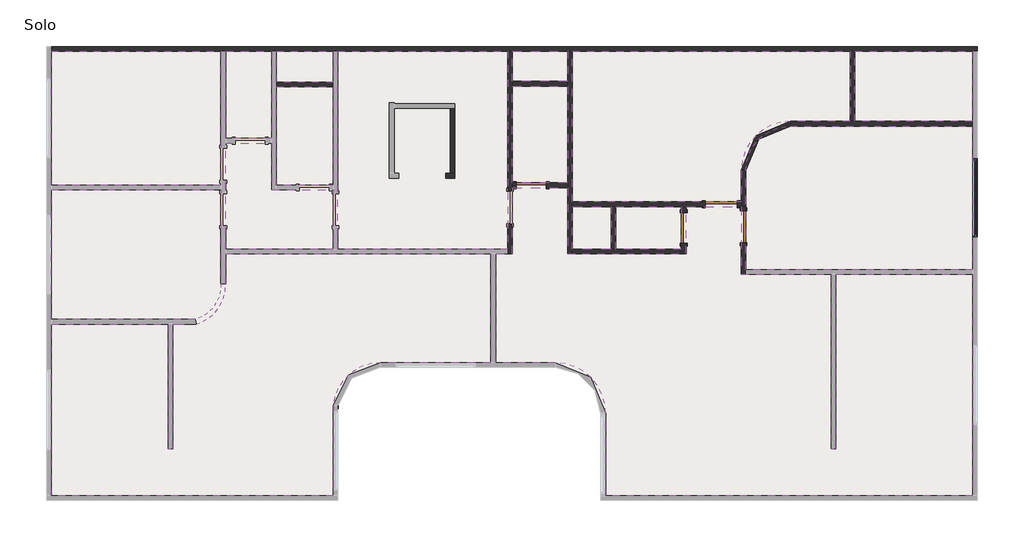
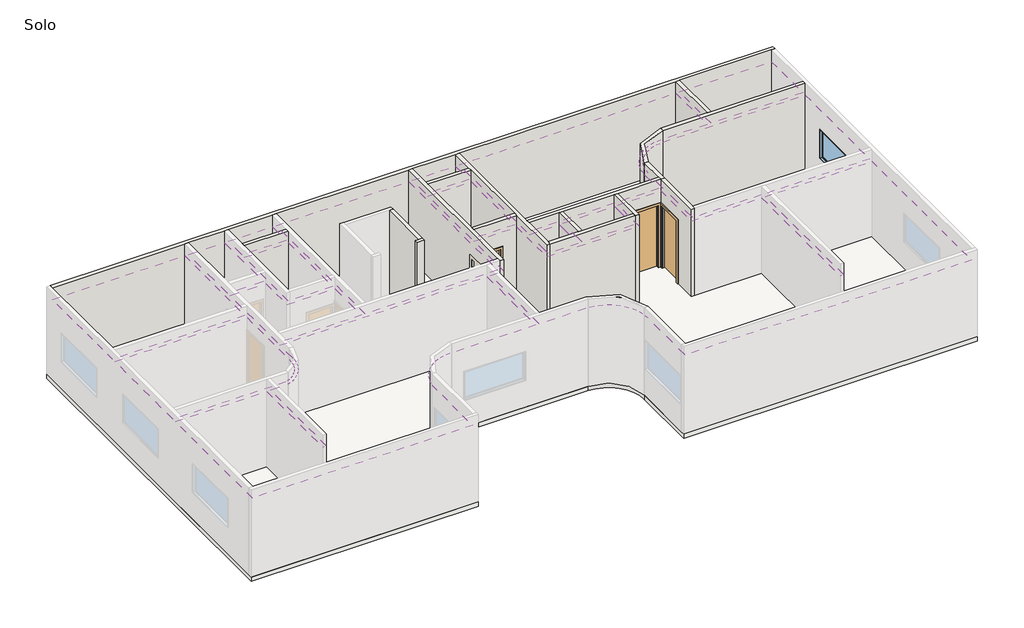
# One storey, part 2 of 2: 17 walls, 16 coverings, 4 doors, 1 slab, 1 window.
"""IFC4 building model written with IfcOpenShell, lengths in millimetres."""

import ifcopenshell
import ifcopenshell.guid

model = None  # the IFC model being written
_history = None  # IfcOwnerHistory: only IFC2X3 demands one
_inside = {}  # id of a spatial element -> (the spatial element, [elements in it])
_under = {}  # id of a project, library or spatial element -> (it, [spatial elements below it])
_declared = {}  # id of a project -> (the project, [libraries it declares])
_typed = {}  # id of a type object -> (the type object, [elements of that type])
_made_of = {}  # id of a material, layer set ... -> (it, [elements and type objects made of it])


def new_model(schema):
    """Start an empty IFC model of exactly this schema.

    Asked for "IFC4X3", IfcOpenShell would pick the latest addendum, in which some entities
    have other attributes; the version numbers below select the first issue.
    IFC2X3 requires an IfcOwnerHistory on every rooted entity: one is made here for all.
    """
    global model, _history
    if schema == "IFC4X3":
        model = ifcopenshell.file(schema_version=(4, 3, 0, 0))
    else:
        model = ifcopenshell.file(schema=schema)
    _inside.clear()
    _under.clear()
    _declared.clear()
    _typed.clear()
    _made_of.clear()
    _history = None
    if model.schema == "IFC2X3":
        org = make("IfcOrganization", Name="unknown")
        user = make(
            "IfcPersonAndOrganization",
            ThePerson=make("IfcPerson", FamilyName="unknown"),
            TheOrganization=org,
        )
        app = make(
            "IfcApplication",
            ApplicationDeveloper=org,
            Version="unknown",
            ApplicationFullName="unknown",
            ApplicationIdentifier="unknown",
        )
        _history = make(
            "IfcOwnerHistory",
            OwningUser=user,
            OwningApplication=app,
            ChangeAction="ADDED",
            CreationDate=0,
        )
    return model


def make(cls, **values):
    """One entity of the class cls with the attributes given. An attribute that is None is left unset."""
    return model.create_entity(
        cls, **{name: value for name, value in values.items() if value is not None}
    )


def rooted(cls, **values):
    """An entity with a GlobalId (a new one), such as an element, a storey or a relation."""
    return make(cls, GlobalId=ifcopenshell.guid.new(), OwnerHistory=_history, **values)


def si_unit(unit_type, name, prefix=None):
    """IfcSIUnit, for example si_unit("LENGTHUNIT", "METRE", prefix="MILLI")."""
    return make("IfcSIUnit", UnitType=unit_type, Prefix=prefix, Name=name)


def assignment(units):
    """IfcUnitAssignment: the units of a project."""
    return None if units is None else make("IfcUnitAssignment", Units=units)


def point(xyz):
    """IfcCartesianPoint."""
    return None if xyz is None else make("IfcCartesianPoint", Coordinates=xyz)


def direction(xyz):
    """IfcDirection."""
    return None if xyz is None else make("IfcDirection", DirectionRatios=xyz)


def frame(location, z_axis=None, x_axis=None):
    """IfcAxis2Placement3D, a coordinate frame: its origin and axes. An axis left out is left unset."""
    return make(
        "IfcAxis2Placement3D",
        Location=point(location),
        Axis=direction(z_axis),
        RefDirection=direction(x_axis),
    )


def frame_2d(location, x_axis=None):
    """IfcAxis2Placement2D, a coordinate frame in the plane: its origin and x axis."""
    return make(
        "IfcAxis2Placement2D", Location=point(location), RefDirection=direction(x_axis)
    )


def origin():
    """The frame at (0, 0, 0) with its axes left unset."""
    return frame((0.0, 0.0, 0.0))


def origin_with_axes():
    """The frame at (0, 0, 0) with the z axis (0, 0, 1) and the x axis (1, 0, 0) written out."""
    return frame((0.0, 0.0, 0.0), z_axis=(0.0, 0.0, 1.0), x_axis=(1.0, 0.0, 0.0))


def place(relative_to, where):
    """IfcLocalPlacement: puts the frame where relative to a parent placement (None: the world)."""
    return make(
        "IfcLocalPlacement", PlacementRelTo=relative_to, RelativePlacement=where
    )


def context(
    kind, dimensions, precision=None, world=None, true_north=None, identifier=None
):
    """IfcGeometricRepresentationContext, for example the 3D "Model" context."""
    return make(
        "IfcGeometricRepresentationContext",
        ContextIdentifier=identifier,
        ContextType=kind,
        CoordinateSpaceDimension=dimensions,
        Precision=precision,
        WorldCoordinateSystem=world,
        TrueNorth=true_north,
    )


def project(units=None, contexts=None):
    """IfcProject with its units and contexts."""
    return rooted(
        "IfcProject",
        Name="project",
        RepresentationContexts=contexts,
        UnitsInContext=assignment(units),
    )


def spatial(cls, under=None, at=None, **own):
    """A site, building, storey or space (cls), placed at a placement, below another one or the project."""
    s = rooted(cls, ObjectPlacement=at, **own)
    if under is not None:
        _under.setdefault(under.id(), (under, []))[1].append(s)
    return s


def polyline(points):
    """IfcPolyline through the points."""
    return make("IfcPolyline", Points=[point(p) for p in points])


def circle_curve(where, radius):
    """IfcCircle in the frame where."""
    return make("IfcCircle", Position=where, Radius=radius)


def trimmed(basis, trim1, trim2, sense, master):
    """IfcTrimmedCurve: the piece of a basis curve between two trims."""
    return make(
        "IfcTrimmedCurve",
        BasisCurve=basis,
        Trim1=trim1,
        Trim2=trim2,
        SenseAgreement=sense,
        MasterRepresentation=master,
    )


def segment(curve, same_sense, transition):
    """IfcCompositeCurveSegment."""
    return make(
        "IfcCompositeCurveSegment",
        Transition=transition,
        SameSense=same_sense,
        ParentCurve=curve,
    )


def composite_curve(segments, self_intersect=None):
    """IfcCompositeCurve: segments joined end to end."""
    return make("IfcCompositeCurve", Segments=segments, SelfIntersect=self_intersect)


def outline(outer, holes=None, kind="AREA"):
    """IfcArbitraryClosedProfileDef: a profile drawn as a closed curve; with holes, ...WithVoids."""
    if holes is None:
        return make("IfcArbitraryClosedProfileDef", ProfileType=kind, OuterCurve=outer)
    return make(
        "IfcArbitraryProfileDefWithVoids",
        ProfileType=kind,
        OuterCurve=outer,
        InnerCurves=holes,
    )


def extrude(swept, where, along, depth):
    """IfcExtrudedAreaSolid: the profile swept, set in the frame where, extruded along a direction by depth."""
    return make(
        "IfcExtrudedAreaSolid",
        SweptArea=swept,
        Position=where,
        ExtrudedDirection=direction(along),
        Depth=depth,
    )


def faces_of(points, faces, orient=None, outer=None):
    """IfcFace entities. A face is a list of loops; a loop is a list of indices into points, from 0.

    orient and outer hold one flag for each loop. By default every Orientation is true, the
    first loop of a face is its IfcFaceOuterBound and the others are IfcFaceBound.
    """
    made = []
    for i, loops in enumerate(faces):
        bounds = []
        for j, loop in enumerate(loops):
            is_outer = j == 0 if outer is None else outer[i][j]
            bounds.append(
                make(
                    "IfcFaceOuterBound" if is_outer else "IfcFaceBound",
                    Bound=make("IfcPolyLoop", Polygon=[points[k] for k in loop]),
                    Orientation=True if orient is None else orient[i][j],
                )
            )
        made.append(make("IfcFace", Bounds=bounds))
    return made


def faceted_brep(points, faces, orient=None, outer=None, voids=None):
    """IfcFacetedBrep: a solid bounded by flat faces; with voids (closed shells), ...WithVoids."""
    shared = [point(p) for p in points]
    hull = make("IfcClosedShell", CfsFaces=faces_of(shared, faces, orient, outer))
    if voids is None:
        return make("IfcFacetedBrep", Outer=hull)
    return make(
        "IfcFacetedBrepWithVoids",
        Outer=hull,
        Voids=[
            make(cls, CfsFaces=faces_of(shared, fs, o, b)) for cls, fs, o, b in voids
        ],
    )


def shape(context_of_items, identifier, shape_type, items):
    """IfcShapeRepresentation: the items that make up one representation, for example the "Body"."""
    return make(
        "IfcShapeRepresentation",
        ContextOfItems=context_of_items,
        RepresentationIdentifier=identifier,
        RepresentationType=shape_type,
        Items=items,
    )


def source(mapping_origin, context_of_items, identifier, shape_type, items):
    """IfcRepresentationMap: a shape defined once, which mapped items show again and again."""
    return make(
        "IfcRepresentationMap",
        MappingOrigin=mapping_origin,
        MappedRepresentation=shape(context_of_items, identifier, shape_type, items),
    )


def transform(
    local_origin,
    x_axis=None,
    y_axis=None,
    z_axis=None,
    scale=None,
    scale2=None,
    scale3=None,
    uniform=True,
):
    """IfcCartesianTransformationOperator3D, or its non-uniform kind. x_axis, y_axis, z_axis: its Axis1, 2, 3."""
    if uniform:
        return make(
            "IfcCartesianTransformationOperator3D",
            Axis1=direction(x_axis),
            Axis2=direction(y_axis),
            LocalOrigin=point(local_origin),
            Scale=scale,
            Axis3=direction(z_axis),
        )
    return make(
        "IfcCartesianTransformationOperator3DnonUniform",
        Axis1=direction(x_axis),
        Axis2=direction(y_axis),
        LocalOrigin=point(local_origin),
        Scale=scale,
        Axis3=direction(z_axis),
        Scale2=scale2,
        Scale3=scale3,
    )


def mapped(mapping_source, mapping_target):
    """IfcMappedItem: shows the shape of a source again, moved by a transform."""
    return make(
        "IfcMappedItem", MappingSource=mapping_source, MappingTarget=mapping_target
    )


def made_of(thing, what):
    """Note that an element or type object is made of a material, layer set ...; save() writes the relation."""
    if what is not None:
        _made_of.setdefault(what.id(), (what, []))[1].append(thing)
    return thing


def element(
    cls,
    number,
    at=None,
    inside=None,
    cuts=None,
    type_object=None,
    material=None,
    context=None,
    identifier="Body",
    shape_type=None,
    held_by="IfcProductDefinitionShape",
    body=None,
    shapes=None,
    **own,
):
    """One element of the class cls, such as IfcWall. Its Tag is "e" and its number.

    at: its placement. inside: the storey or other place that contains it. cuts: it is an
    opening in that element (IfcRelVoidsElement). A single representation is given by context,
    identifier, shape_type and body (its items); several are given by shapes. held_by: the class
    of the entity that holds the representations. save() writes the other relations.
    """
    e = rooted(cls, Tag="e%d" % number, ObjectPlacement=at, **own)
    if body is not None:
        shapes = [shape(context, identifier, shape_type, body)]
    if shapes is not None:
        e.Representation = make(held_by, Representations=shapes)
    if inside is not None:
        _inside.setdefault(inside.id(), (inside, []))[1].append(e)
    if cuts is not None:
        rooted(
            "IfcRelVoidsElement", RelatingBuildingElement=cuts, RelatedOpeningElement=e
        )
    if type_object is not None:
        _typed.setdefault(type_object.id(), (type_object, []))[1].append(e)
    return made_of(e, material)


def aggregate(whole, parts):
    """IfcRelAggregates: a whole, such as a stair, and the parts it consists of."""
    return rooted("IfcRelAggregates", RelatingObject=whole, RelatedObjects=parts)


def save(model, path):
    """Write the relations noted so far, then the file.

    IfcRelAggregates (storeys below a building ...), IfcRelContainedInSpatialStructure (elements
    in a storey), IfcRelDefinesByType, IfcRelAssociatesMaterial and IfcRelDeclares: one each for
    every whole, place, type object, material and project.
    """
    for whole, parts in _under.values():
        aggregate(whole, parts)
    for where, things in _inside.values():
        rooted(
            "IfcRelContainedInSpatialStructure",
            RelatedElements=things,
            RelatingStructure=where,
        )
    for kind, things in _typed.values():
        rooted("IfcRelDefinesByType", RelatedObjects=things, RelatingType=kind)
    for what, things in _made_of.values():
        rooted("IfcRelAssociatesMaterial", RelatedObjects=things, RelatingMaterial=what)
    for by, libraries in _declared.values():
        rooted("IfcRelDeclares", RelatingContext=by, RelatedDefinitions=libraries)
    model.write(path)


def door_0762_x_2032mm_ca16c8eb(model_context):
    return source(origin(), model_context, "Body", "SweptSolid", [
        extrude(outline(polyline([(2108.0, -457.0), (0.0, -457.0), (0.0, -381.0), (2032.0, -381.0), (2032.0, 381.0), (0.0, 381.0), (0.0, 457.0), (2108.0, 457.0), (2108.0, -457.0)])), frame((0.0, 60.0, 0.0), z_axis=(0.0, 1.0, 0.0), x_axis=(0.0, 0.0, 1.0)), (0.0, 0.0, 1.0), 25.0),
        extrude(outline(polyline([(2108.0, 457.0), (2108.0, -457.0), (0.0, -457.0), (0.0, -381.0), (2032.0, -381.0), (2032.0, 381.0), (0.0, 381.0), (0.0, 457.0), (2108.0, 457.0)])), frame((0.0, -85.0, 0.0), z_axis=(0.0, 1.0, 0.0), x_axis=(0.0, 0.0, 1.0)), (0.0, 0.0, 1.0), 25.0),
        extrude(outline(polyline([(381.0, 9.0), (-381.0, 9.0), (-381.0, 60.0), (381.0, 60.0), (381.0, 9.0)])), origin_with_axes(), (0.0, 0.0, 1.0), 2032.0),
    ])


def door_0762_x_2032mm_5282416c(model_context):
    return source(origin(), model_context, "Body", "SweptSolid", [
        extrude(outline(polyline([(2108.0, -457.0), (0.0, -457.0), (0.0, -381.0), (2032.0, -381.0), (2032.0, 381.0), (0.0, 381.0), (0.0, 457.0), (2108.0, 457.0), (2108.0, -457.0)])), frame((0.0, -85.0, 0.0), z_axis=(0.0, 1.0, 0.0), x_axis=(0.0, 0.0, 1.0)), (0.0, 0.0, 1.0), 25.0),
        extrude(outline(polyline([(2108.0, 457.0), (2108.0, -457.0), (0.0, -457.0), (0.0, -381.0), (2032.0, -381.0), (2032.0, 381.0), (0.0, 381.0), (0.0, 457.0), (2108.0, 457.0)])), frame((0.0, 60.0, 0.0), z_axis=(0.0, 1.0, 0.0), x_axis=(0.0, 0.0, 1.0)), (0.0, 0.0, 1.0), 25.0),
        extrude(outline(polyline([(381.0, -9.0), (381.0, -60.0), (-381.0, -60.0), (-381.0, -9.0), (381.0, -9.0)])), origin_with_axes(), (0.0, 0.0, 1.0), 2032.0),
    ])


def door_0813_x_2134mm_314d41b2(model_context):
    return source(origin(), model_context, "Body", "SweptSolid", [
        extrude(outline(polyline([(2210.0, -482.5), (0.0, -482.5), (0.0, -406.5), (2134.0, -406.5), (2134.0, 406.5), (0.0, 406.5), (0.0, 482.5), (2210.0, 482.5), (2210.0, -482.5)])), frame((0.0, 60.0, 0.0), z_axis=(0.0, 1.0, 0.0), x_axis=(0.0, 0.0, 1.0)), (0.0, 0.0, 1.0), 25.0),
        extrude(outline(polyline([(2210.0, 482.5), (2210.0, -482.5), (0.0, -482.5), (0.0, -406.5), (2134.0, -406.5), (2134.0, 406.5), (0.0, 406.5), (0.0, 482.5), (2210.0, 482.5)])), frame((0.0, -85.0, 0.0), z_axis=(0.0, 1.0, 0.0), x_axis=(0.0, 0.0, 1.0)), (0.0, 0.0, 1.0), 25.0),
        extrude(outline(polyline([(406.5, 9.0), (-406.5, 9.0), (-406.5, 60.0), (406.5, 60.0), (406.5, 9.0)])), origin_with_axes(), (0.0, 0.0, 1.0), 2134.0),
    ])


def m_fixo_2000_x_1000mm_897e8a61(model_context):
    return source(origin(), model_context, "Body", "SweptSolid", [
        extrude(outline(polyline([(-937.0, 38.0), (937.0, 38.0), (937.0, 26.0), (-937.0, 26.0), (-937.0, 38.0)])), frame((0.0, 0.0, 978.0), z_axis=(0.0, 0.0, 1.0), x_axis=(1.0, 0.0, 0.0)), (0.0, 0.0, 1.0), 874.0),
        extrude(outline(polyline([(1896.0, -981.0), (934.0, -981.0), (934.0, 981.0), (1896.0, 981.0), (1896.0, -981.0)]), holes=[polyline([(1852.0, -937.0), (1852.0, 937.0), (978.0, 937.0), (978.0, -937.0), (1852.0, -937.0)])]), frame((0.0, 10.0, 0.0), z_axis=(0.0, 1.0, 0.0), x_axis=(0.0, 0.0, 1.0)), (0.0, 0.0, 1.0), 44.0),
        extrude(outline(polyline([(1915.0, -1000.0), (915.0, -1000.0), (915.0, 1000.0), (1915.0, 1000.0), (1915.0, -1000.0)]), holes=[polyline([(1896.0, -981.0), (1896.0, 981.0), (934.0, 981.0), (934.0, -981.0), (1896.0, -981.0)])]), frame((0.0, 10.0, 0.0), z_axis=(0.0, 1.0, 0.0), x_axis=(0.0, 0.0, 1.0)), (0.0, 0.0, 1.0), 63.0),
        extrude(outline(polyline([(1915.0, -1000.0), (915.0, -1000.0), (915.0, 1000.0), (1915.0, 1000.0), (1915.0, -1000.0)]), holes=[polyline([(1883.0, -968.0), (1883.0, 968.0), (947.0, 968.0), (947.0, -968.0), (1883.0, -968.0)])]), frame((0.0, -47.0, 0.0), z_axis=(0.0, 1.0, 0.0), x_axis=(0.0, 0.0, 1.0)), (0.0, 0.0, 1.0), 57.0),
    ])


model = new_model("IFC4")

# Units and contexts
model_context = context("Model", 3, world=origin())
ifc_project = project(units=[si_unit("LENGTHUNIT", "METRE", prefix="MILLI")], contexts=[model_context])

# Site, building, storey
site = spatial("IfcSite", under=ifc_project)
building = spatial("IfcBuilding", under=site)
storey = spatial("IfcBuildingStorey", under=building, Name="Solo", Elevation=0.0)

# Coverings
placement = place(None, origin())
element("IfcCovering", 1, ObjectType="Simples", at=placement, inside=storey, context=model_context, shape_type="SweptSolid", body=[
    extrude(outline(polyline([(-7687.5462561, 5315.4313177), (-7687.5462561, 1920.3975855), (-11987.7424597, 1920.3975855), (-11987.7424597, 5315.4313177), (-7687.5462561, 5315.4313177)])), frame((0.0, 0.0, 2600.0), z_axis=(0.0, 0.0, 1.0), x_axis=(1.0, 0.0, 0.0)), (0.0, 0.0, 1.0), 57.0),
])
element("IfcCovering", 2, ObjectType="Simples", at=placement, inside=storey, context=model_context, shape_type="SweptSolid", body=[
    extrude(outline(polyline([(-7567.5462561, 3105.4313177), (-7567.5462561, 5315.4313177), (-6397.5462561, 5315.4313177), (-6397.5462561, 3105.4313177), (-7567.5462561, 3105.4313177)])), frame((0.0, 0.0, 2600.0), z_axis=(0.0, 0.0, 1.0), x_axis=(1.0, 0.0, 0.0)), (0.0, 0.0, 1.0), 57.0),
])
element("IfcCovering", 3, ObjectType="Simples", at=placement, inside=storey, context=model_context, shape_type="SweptSolid", body=[
    extrude(outline(polyline([(-4837.5462561, 293.7558339), (-7567.5462561, 293.7558339), (-7567.5462561, 2985.4313177), (-6397.5462561, 2985.4313177), (-6397.5462561, 1800.3975855), (-4837.5462561, 1800.3975855), (-4837.5462561, 293.7558339)])), frame((0.0, 0.0, 2600.0), z_axis=(0.0, 0.0, 1.0), x_axis=(1.0, 0.0, 0.0)), (0.0, 0.0, 1.0), 57.0),
])
element("IfcCovering", 4, ObjectType="Simples", at=placement, inside=storey, context=model_context, shape_type="SweptSolid", body=[
    extrude(outline(polyline([(-6277.5462561, 1920.3975855), (-6277.5462561, 4409.8633053), (-4837.5462561, 4409.8633053), (-4837.5462561, 1920.3975855), (-6277.5462561, 1920.3975855)])), frame((0.0, 0.0, 2600.0), z_axis=(0.0, 0.0, 1.0), x_axis=(1.0, 0.0, 0.0)), (0.0, 0.0, 1.0), 57.0),
])
element("IfcCovering", 5, ObjectType="Simples", at=placement, inside=storey, context=model_context, shape_type="SweptSolid", body=[
    extrude(outline(polyline([(-6277.5462561, 4529.8633053), (-6277.5462561, 5315.4313177), (-4837.5462561, 5315.4313177), (-4837.5462561, 4529.8633053), (-6277.5462561, 4529.8633053)])), frame((0.0, 0.0, 2600.0), z_axis=(0.0, 0.0, 1.0), x_axis=(1.0, 0.0, 0.0)), (0.0, 0.0, 1.0), 57.0),
])
element("IfcCovering", 6, ObjectType="Simples", at=placement, inside=storey, context=model_context, shape_type="SweptSolid", body=[
    extrude(outline(composite_curve([segment(polyline([(-7687.5462561, 1800.3975855), (-7687.5462561, -585.6507938)]), True, "CONTINUOUS"), segment(trimmed(circle_curve(frame_2d((-8591.3131194, -617.7595428)), 904.3370583), [point((-7687.5462561, -585.6507938))], [point((-8333.6137775, -1484.6024145))], False, "CARTESIAN"), True, "CONTINUOUS"), segment(polyline([(-8333.6137775, -1484.6024145), (-11987.7424597, -1484.6024145), (-11987.7424597, 1800.3975855), (-7687.5462561, 1800.3975855)]), True, "CONTINUOUS")], self_intersect=False)), frame((0.0, 0.0, 2600.0), z_axis=(0.0, 0.0, 1.0), x_axis=(1.0, 0.0, 0.0)), (0.0, 0.0, 1.0), 57.0),
])
element("IfcCovering", 7, ObjectType="Simples", at=placement, inside=storey, context=model_context, shape_type="SweptSolid", body=[
    extrude(outline(composite_curve([segment(trimmed(circle_curve(frame_2d((-8591.3131194, -617.7595428)), 1024.3370583), [point((-8316.7087575, -1604.6024145))], [point((-7567.5462561, -583.5861825))], True, "CARTESIAN"), True, "CONTINUOUS"), segment(polyline([(-7567.5462561, -583.5861825), (-7567.5462561, 173.7558339), (-837.607531, 173.7558339), (-837.607531, -2583.6287272), (-3639.3298266, -2583.6287272)]), True, "CONTINUOUS"), segment(trimmed(circle_curve(frame_2d((-3640.8284375, -3788.2857678)), 1204.6579727), [point((-3639.3298266, -2583.6287272))], [point((-4839.3676237, -3667.0230345))], True, "CARTESIAN"), True, "CONTINUOUS"), segment(polyline([(-4839.3676237, -3667.0230345), (-4839.3676237, -5954.8147341), (-11987.7424597, -5954.8147341), (-11987.7424597, -1604.6024145), (-9023.1250641, -1604.6024145), (-9023.1250641, -4764.547347), (-8903.1250641, -4764.547347), (-8903.1250641, -1604.6024145), (-8316.7087575, -1604.6024145)]), True, "CONTINUOUS")], self_intersect=False)), frame((0.0, 0.0, 2600.0), z_axis=(0.0, 0.0, 1.0), x_axis=(1.0, 0.0, 0.0)), (0.0, 0.0, 1.0), 57.0),
])
element("IfcCovering", 8, ObjectType="Simples", at=placement, inside=storey, context=model_context, shape_type="SweptSolid", body=[
    extrude(outline(polyline([(-4717.5462561, 5315.4313177), (-410.3138992, 5315.4313177), (-410.3138992, 293.7558339), (-4717.5462561, 293.7558339), (-4717.5462561, 5315.4313177)]), holes=[polyline([(-3409.5233936, 2098.2818001), (-3170.7928649, 2098.2818001), (-3170.7928649, 2218.2818001), (-3289.5233936, 2218.2818001), (-3289.5233936, 3869.8633053), (-1870.3138992, 3869.8633053), (-1870.3138992, 2218.2818001), (-1979.2560065, 2218.2818001), (-1979.2560065, 2098.2818001), (-1750.3138992, 2098.2818001), (-1750.3138992, 3989.8633053), (-3409.5233936, 3989.8633053), (-3409.5233936, 2098.2818001)])]), frame((0.0, 0.0, 2600.0), z_axis=(0.0, 0.0, 1.0), x_axis=(1.0, 0.0, 0.0)), (0.0, 0.0, 1.0), 57.0),
])
element("IfcCovering", 9, ObjectType="Simples", at=placement, inside=storey, context=model_context, shape_type="SweptSolid", body=[
    extrude(outline(polyline([(1109.6861008, 1979.9744284), (-290.3138992, 1979.9744284), (-290.3138992, 4429.8633053), (1109.6861008, 4429.8633053), (1109.6861008, 1979.9744284)])), frame((0.0, 0.0, 2600.0), z_axis=(0.0, 0.0, 1.0), x_axis=(1.0, 0.0, 0.0)), (0.0, 0.0, 1.0), 57.0),
])
element("IfcCovering", 10, ObjectType="Simples", at=placement, inside=storey, context=model_context, shape_type="SweptSolid", body=[
    extrude(outline(polyline([(-290.3138992, 4549.8633053), (-290.3138992, 5315.4313177), (1109.6861008, 5315.4313177), (1109.6861008, 4549.8633053), (-290.3138992, 4549.8633053)])), frame((0.0, 0.0, 2600.0), z_axis=(0.0, 0.0, 1.0), x_axis=(1.0, 0.0, 0.0)), (0.0, 0.0, 1.0), 57.0),
])
element("IfcCovering", 11, ObjectType="Simples", at=placement, inside=storey, context=model_context, shape_type="SweptSolid", body=[
    extrude(outline(composite_curve([segment(polyline([(7912.4537439, -340.1148653), (11383.1038545, -340.1148653), (11383.1038545, -5955.2378912), (2072.392469, -5955.2378912), (2072.392469, -3863.6287272)]), True, "CONTINUOUS"), segment(trimmed(circle_curve(frame_2d((792.392469, -3863.6287272)), 1280.0), [point((2072.392469, -3863.6287272))], [point((792.392469, -2583.6287272))], True, "CARTESIAN"), True, "CONTINUOUS"), segment(polyline([(792.392469, -2583.6287272), (-717.607531, -2583.6287272), (-717.607531, 173.7558339), (-290.3138992, 173.7558339), (-290.3138992, 1859.9744284), (1109.6861008, 1859.9744284), (1109.6861008, 173.7558339), (4112.4537439, 173.7558339), (4112.4537439, 1373.1481066), (5512.4537439, 1373.1481066), (5512.4537439, -340.1148653), (7792.4537439, -340.1148653), (7792.4537439, -4764.547347), (7912.4537439, -4764.547347), (7912.4537439, -340.1148653)]), True, "CONTINUOUS")], self_intersect=False)), frame((0.0, 0.0, 2600.0), z_axis=(0.0, 0.0, 1.0), x_axis=(1.0, 0.0, 0.0)), (0.0, 0.0, 1.0), 57.0),
])
element("IfcCovering", 12, ObjectType="Simples", at=placement, inside=storey, context=model_context, shape_type="SweptSolid", body=[
    extrude(outline(polyline([(2209.6861008, 293.7558339), (1229.6861008, 293.7558339), (1229.6861008, 1373.1481066), (2209.6861008, 1373.1481066), (2209.6861008, 293.7558339)])), frame((0.0, 0.0, 2600.0), z_axis=(0.0, 0.0, 1.0), x_axis=(1.0, 0.0, 0.0)), (0.0, 0.0, 1.0), 57.0),
])
element("IfcCovering", 13, ObjectType="Simples", at=placement, inside=storey, context=model_context, shape_type="SweptSolid", body=[
    extrude(outline(polyline([(3992.4537439, 1373.1481066), (3992.4537439, 293.7558339), (2329.6861008, 293.7558339), (2329.6861008, 1373.1481066), (3992.4537439, 1373.1481066)])), frame((0.0, 0.0, 2600.0), z_axis=(0.0, 0.0, 1.0), x_axis=(1.0, 0.0, 0.0)), (0.0, 0.0, 1.0), 57.0),
])
element("IfcCovering", 14, ObjectType="Simples", at=placement, inside=storey, context=model_context, shape_type="SweptSolid", body=[
    extrude(outline(composite_curve([segment(polyline([(6754.736955, 3415.4313177), (11383.1038545, 3415.4313177), (11383.1038545, -220.1148653), (5632.4537439, -220.1148653), (5632.4537439, 1433.1481066), (5632.4537439, 2293.1481066)]), True, "CONTINUOUS"), segment(trimmed(circle_curve(frame_2d((6754.736955, 2293.1481066)), 1122.2832111), [point((5632.4537439, 2293.1481066))], [point((6754.736955, 3415.4313177))], False, "CARTESIAN"), True, "CONTINUOUS")], self_intersect=False)), frame((0.0, 0.0, 2600.0), z_axis=(0.0, 0.0, 1.0), x_axis=(1.0, 0.0, 0.0)), (0.0, 0.0, 1.0), 57.0),
])
element("IfcCovering", 15, ObjectType="Simples", at=placement, inside=storey, context=model_context, shape_type="SweptSolid", body=[
    extrude(outline(polyline([(8392.4537439, 5315.4313177), (11383.1038545, 5315.4313177), (11383.1038545, 3535.4313177), (8392.4537439, 3535.4313177), (8392.4537439, 5315.4313177)])), frame((0.0, 0.0, 2600.0), z_axis=(0.0, 0.0, 1.0), x_axis=(1.0, 0.0, 0.0)), (0.0, 0.0, 1.0), 57.0),
])
element("IfcCovering", 16, ObjectType="Simples", at=placement, inside=storey, context=model_context, shape_type="SweptSolid", body=[
    extrude(outline(composite_curve([segment(polyline([(1229.6861008, 1493.1481066), (1229.6861008, 5315.4313177), (8272.4537439, 5315.4313177), (8272.4537439, 3535.4313177), (6754.736955, 3535.4313177)]), True, "CONTINUOUS"), segment(trimmed(circle_curve(frame_2d((6754.736955, 2293.1481066)), 1242.2832111), [point((6754.736955, 3535.4313177))], [point((5512.4537439, 2293.1481066))], True, "CARTESIAN"), True, "CONTINUOUS"), segment(polyline([(5512.4537439, 2293.1481066), (5512.4537439, 1493.1481066), (1229.6861008, 1493.1481066)]), True, "CONTINUOUS")], self_intersect=False)), frame((0.0, 0.0, 2600.0), z_axis=(0.0, 0.0, 1.0), x_axis=(1.0, 0.0, 0.0)), (0.0, 0.0, 1.0), 57.0),
])

# Doors
door_0762_x_2032mm_shape = door_0762_x_2032mm_ca16c8eb(model_context)
element("IfcDoor", 17, ObjectType="M_Folha única : 0762 x 2032mm", at=placement, inside=storey, context=model_context, shape_type="MappedRepresentation", body=[
    mapped(door_0762_x_2032mm_shape, transform((4052.4537439, 833.4519702, 0.0), x_axis=(0.0, 1.0, 0.0), y_axis=(-1.0, 0.0, 0.0), z_axis=(0.0, 0.0, 1.0))),
])
door_0762_x_2032mm_2_shape = door_0762_x_2032mm_5282416c(model_context)
element("IfcDoor", 18, ObjectType="M_Folha única : 0762 x 2032mm", at=placement, inside=storey, context=model_context, shape_type="MappedRepresentation", body=[
    mapped(door_0762_x_2032mm_2_shape, transform((190.6861008, 1919.9744284, 0.0), x_axis=(-1.0, 0.0, 0.0), y_axis=(0.0, -1.0, 0.0), z_axis=(0.0, 0.0, 1.0))),
])
door_0813_x_2134mm_shape = door_0813_x_2134mm_314d41b2(model_context)
element("IfcDoor", 19, ObjectType="M_Folha única : 0813 x 2134mm", at=placement, inside=storey, context=model_context, shape_type="MappedRepresentation", body=[
    mapped(door_0813_x_2134mm_shape, transform((5005.9537439, 1433.1481066, 0.0), x_axis=(1.0, 0.0, 0.0), y_axis=(0.0, 1.0, 0.0), z_axis=(0.0, 0.0, 1.0))),
])
element("IfcDoor", 20, ObjectType="M_Folha única : 0813 x 2134mm", at=placement, inside=storey, context=model_context, shape_type="MappedRepresentation", body=[
    mapped(door_0813_x_2134mm_shape, transform((5572.4537439, 866.6481066, 0.0), x_axis=(0.0, -1.0, 0.0), y_axis=(1.0, 0.0, 0.0), z_axis=(0.0, 0.0, 1.0))),
])

# Slab
element("IfcSlab", 21, ObjectType="Genérico 150 mm", at=placement, inside=storey, context=model_context, shape_type="SweptSolid", body=[
    extrude(outline(composite_curve([segment(polyline([(11503.1038545, 5435.4313177), (11503.1038545, -6075.2378912), (1952.392469, -6075.2378912), (1952.392469, -3863.6287272)]), True, "CONTINUOUS"), segment(trimmed(circle_curve(frame_2d((792.392469, -3863.6287272)), 1160.0), [point((1952.392469, -3863.6287272))], [point((792.392469, -2703.6287272))], True, "CARTESIAN"), True, "CONTINUOUS"), segment(polyline([(792.392469, -2703.6287272), (-3239.2179842, -2703.6287272)]), True, "CONTINUOUS"), segment(trimmed(circle_curve(frame_2d((-3563.9668473, -3812.4520359)), 1155.4007764), [point((-3239.2179842, -2703.6287272))], [point((-4719.3676237, -3812.4520359))], True, "CARTESIAN"), True, "CONTINUOUS"), segment(polyline([(-4719.3676237, -3812.4520359), (-4719.3676237, -6075.2378912), (-12107.7424597, -6075.2378912), (-12107.7424597, 5435.4313177), (11503.1038545, 5435.4313177)]), True, "CONTINUOUS")], self_intersect=False)), frame((0.0, 0.0, -150.0), z_axis=(0.0, 0.0, 1.0), x_axis=(1.0, 0.0, 0.0)), (0.0, 0.0, 1.0), 150.0),
])

# Walls
element("IfcWall", 22, ObjectType="Genérico - 120 mm - Preenchido 2", at=placement, inside=storey, context=model_context, shape_type="Brep", body=[
    faceted_brep([(-11987.7424597, 5315.4313177, 0.0), (-7687.5462561, 5315.4313177, 0.0), (-7567.5462561, 5315.4313177, 0.0), (-6397.5462561, 5315.4313177, 0.0), (-6277.5462561, 5315.4313177, 0.0), (-4837.5462561, 5315.4313177, 0.0), (-4717.5462561, 5315.4313177, 0.0), (-410.3138992, 5315.4313177, 0.0), (-290.3138992, 5315.4313177, 0.0), (1109.6861008, 5315.4313177, 0.0), (1229.6861008, 5315.4313177, 0.0), (8272.4537439, 5315.4313177, 0.0), (8392.4537439, 5315.4313177, 0.0), (11383.1038545, 5315.4313177, 0.0), (11503.1038545, 5315.4313177, 0.0), (11503.1038545, 5315.4313177, 3000.0), (11383.1038545, 5315.4313177, 3000.0), (8392.4537439, 5315.4313177, 3000.0), (8272.4537439, 5315.4313177, 3000.0), (1229.6861008, 5315.4313177, 3000.0), (1109.6861008, 5315.4313177, 3000.0), (-290.3138992, 5315.4313177, 3000.0), (-410.3138992, 5315.4313177, 3000.0), (-4717.5462561, 5315.4313177, 3000.0), (-4837.5462561, 5315.4313177, 3000.0), (-6277.5462561, 5315.4313177, 3000.0), (-6397.5462561, 5315.4313177, 3000.0), (-7567.5462561, 5315.4313177, 3000.0), (-7687.5462561, 5315.4313177, 3000.0), (-11987.7424597, 5315.4313177, 3000.0), (-11987.7424597, 5435.4313177, 0.0), (-11987.7424597, 5435.4313177, 3000.0), (11503.1038545, 5435.4313177, 3000.0), (11503.1038545, 5435.4313177, 0.0)], [[[0, 1, 2, 3, 4, 5, 6, 7, 8, 9, 10, 11, 12, 13, 14, 15, 16, 17, 18, 19, 20, 21, 22, 23, 24, 25, 26, 27, 28, 29]], [[30, 31, 32, 33]], [[14, 13, 12, 11, 10, 9, 8, 7, 6, 5, 4, 3, 2, 1, 0, 30, 33]], [[29, 28, 27, 26, 25, 24, 23, 22, 21, 20, 19, 18, 17, 16, 15, 32, 31]], [[15, 14, 33, 32]], [[0, 29, 31, 30]]]),
])
element("IfcWall", 23, ObjectType="Genérico - 120 mm - Preenchido 2", at=placement, inside=storey, context=model_context, shape_type="SweptSolid", body=[
    extrude(outline(polyline([(-6277.5462561, 4529.8633053), (-4837.5462561, 4529.8633053), (-4837.5462561, 4409.8633053), (-6277.5462561, 4409.8633053), (-6277.5462561, 4529.8633053)])), origin_with_axes(), (0.0, 0.0, 1.0), 3000.0),
])
element("IfcWall", 24, ObjectType="Genérico - 120 mm - Preenchido 2", at=placement, inside=storey, context=model_context, shape_type="SweptSolid", body=[
    extrude(outline(polyline([(-1870.3138992, 2218.2818001), (-1870.3138992, 3869.8633053), (-1750.3138992, 3869.8633053), (-1750.3138992, 2218.2818001), (-1870.3138992, 2218.2818001)])), origin_with_axes(), (0.0, 0.0, 1.0), 3000.0),
])
element("IfcWall", 25, ObjectType="Genérico - 120 mm - Preenchido 2", at=placement, inside=storey, context=model_context, shape_type="Brep", body=[
    faceted_brep([(-1750.3138992, 2218.2818001, 0.0), (-1870.3138992, 2218.2818001, 0.0), (-1979.2560065, 2218.2818001, 0.0), (-1979.2560065, 2218.2818001, 3000.0), (-1870.3138992, 2218.2818001, 3000.0), (-1750.3138992, 2218.2818001, 3000.0), (-1750.3138992, 2098.2818001, 0.0), (-1750.3138992, 2098.2818001, 3000.0), (-1979.2560065, 2098.2818001, 3000.0), (-1979.2560065, 2098.2818001, 0.0)], [[[0, 1, 2, 3, 4, 5]], [[6, 7, 8, 9]], [[2, 1, 0, 6, 9]], [[3, 2, 9, 8]], [[5, 4, 3, 8, 7]], [[0, 5, 7, 6]]]),
])
element("IfcWall", 26, ObjectType="Genérico - 120 mm - Preenchido 2", at=placement, inside=storey, context=model_context, shape_type="Brep", body=[
    faceted_brep([(-410.3138992, 5315.4313177, 0.0), (-410.3138992, 1759.9744284, 0.0), (-410.3138992, 1759.9744284, 2134.0), (-410.3138992, 946.9744284, 2134.0), (-410.3138992, 946.9744284, 0.0), (-410.3138992, 293.7558339, 0.0), (-410.3138992, 173.7558339, 0.0), (-410.3138992, 173.7558339, 3000.0), (-410.3138992, 293.7558339, 3000.0), (-410.3138992, 5315.4313177, 3000.0), (-290.3138992, 1759.9744284, 2134.0), (-290.3138992, 1759.9744284, 0.0), (-290.3138992, 1859.9744284, 0.0), (-290.3138992, 1979.9744284, 0.0), (-290.3138992, 4429.8633053, 0.0), (-290.3138992, 4549.8633053, 0.0), (-290.3138992, 5315.4313177, 0.0), (-290.3138992, 5315.4313177, 3000.0), (-290.3138992, 4549.8633053, 3000.0), (-290.3138992, 4429.8633053, 3000.0), (-290.3138992, 1979.9744284, 3000.0), (-290.3138992, 1859.9744284, 3000.0), (-290.3138992, 173.7558339, 3000.0), (-290.3138992, 173.7558339, 0.0), (-290.3138992, 946.9744284, 0.0), (-290.3138992, 946.9744284, 2134.0)], [[[0, 1, 2, 3, 4, 5, 6, 7, 8, 9]], [[10, 11, 12, 13, 14, 15, 16, 17, 18, 19, 20, 21, 22, 23, 24, 25]], [[24, 23, 6, 5, 4]], [[16, 15, 14, 13, 12, 11, 1, 0]], [[9, 8, 7, 22, 21, 20, 19, 18, 17]], [[0, 9, 17, 16]], [[7, 6, 23, 22]], [[2, 1, 11, 10]], [[3, 2, 10, 25]], [[4, 3, 25, 24]]]),
])
element("IfcWall", 27, ObjectType="Genérico - 120 mm - Preenchido 2", at=placement, inside=storey, context=model_context, shape_type="SweptSolid", body=[
    extrude(outline(polyline([(0.0, -290.3138992), (0.0, -190.3138992), (2032.0, -190.3138992), (2032.0, 571.6861008), (0.0, 571.6861008), (0.0, 1109.6861008), (3000.0, 1109.6861008), (3000.0, -290.3138992), (0.0, -290.3138992)])), frame((0.0, 1859.9744284, 0.0), z_axis=(0.0, 1.0, 0.0), x_axis=(0.0, 0.0, 1.0)), (0.0, 0.0, 1.0), 120.0),
])
element("IfcWall", 28, ObjectType="Genérico - 120 mm - Preenchido 2", at=placement, inside=storey, context=model_context, shape_type="SweptSolid", body=[
    extrude(outline(polyline([(1109.6861008, 4429.8633053), (-290.3138992, 4429.8633053), (-290.3138992, 4549.8633053), (1109.6861008, 4549.8633053), (1109.6861008, 4429.8633053)])), origin_with_axes(), (0.0, 0.0, 1.0), 3000.0),
])
element("IfcWall", 29, ObjectType="Genérico - 120 mm - Preenchido 2", at=placement, inside=storey, context=model_context, shape_type="Brep", body=[
    faceted_brep([(1109.6861008, 5315.4313177, 0.0), (1109.6861008, 4549.8633053, 0.0), (1109.6861008, 4429.8633053, 0.0), (1109.6861008, 1979.9744284, 0.0), (1109.6861008, 1859.9744284, 0.0), (1109.6861008, 173.7558339, 0.0), (1109.6861008, 173.7558339, 3000.0), (1109.6861008, 1859.9744284, 3000.0), (1109.6861008, 1979.9744284, 3000.0), (1109.6861008, 4429.8633053, 3000.0), (1109.6861008, 4549.8633053, 3000.0), (1109.6861008, 5315.4313177, 3000.0), (1229.6861008, 5315.4313177, 0.0), (1229.6861008, 5315.4313177, 3000.0), (1229.6861008, 1493.1481066, 3000.0), (1229.6861008, 1373.1481066, 3000.0), (1229.6861008, 293.7558339, 3000.0), (1229.6861008, 173.7558339, 3000.0), (1229.6861008, 173.7558339, 0.0), (1229.6861008, 293.7558339, 0.0), (1229.6861008, 1373.1481066, 0.0), (1229.6861008, 1493.1481066, 0.0)], [[[0, 1, 2, 3, 4, 5, 6, 7, 8, 9, 10, 11]], [[12, 13, 14, 15, 16, 17, 18, 19, 20, 21]], [[5, 4, 3, 2, 1, 0, 12, 21, 20, 19, 18]], [[11, 10, 9, 8, 7, 6, 17, 16, 15, 14, 13]], [[0, 11, 13, 12]], [[6, 5, 18, 17]]]),
])
element("IfcWall", 30, ObjectType="Genérico - 120 mm - Preenchido 2", at=placement, inside=storey, context=model_context, shape_type="Brep", body=[
    faceted_brep([(1229.6861008, 173.7558339, 0.0), (3992.4537439, 173.7558339, 0.0), (3992.4537439, 173.7558339, 3000.0), (1229.6861008, 173.7558339, 3000.0), (1229.6861008, 293.7558339, 0.0), (1229.6861008, 293.7558339, 3000.0), (2209.6861008, 293.7558339, 3000.0), (2329.6861008, 293.7558339, 3000.0), (3992.4537439, 293.7558339, 3000.0), (3992.4537439, 293.7558339, 0.0), (2329.6861008, 293.7558339, 0.0), (2209.6861008, 293.7558339, 0.0)], [[[0, 1, 2, 3]], [[4, 5, 6, 7, 8, 9, 10, 11]], [[1, 0, 4, 11, 10, 9]], [[3, 2, 8, 7, 6, 5]], [[0, 3, 5, 4]], [[2, 1, 9, 8]]]),
])
element("IfcWall", 31, ObjectType="Genérico - 120 mm - Preenchido 2", at=placement, inside=storey, context=model_context, shape_type="Brep", body=[
    faceted_brep([(5412.4537439, 1373.1481066, 2134.0), (5412.4537439, 1373.1481066, 0.0), (5512.4537439, 1373.1481066, 0.0), (5512.4537439, 1373.1481066, 3000.0), (4112.4537439, 1373.1481066, 3000.0), (3992.4537439, 1373.1481066, 3000.0), (2329.6861008, 1373.1481066, 3000.0), (2209.6861008, 1373.1481066, 3000.0), (1229.6861008, 1373.1481066, 3000.0), (1229.6861008, 1373.1481066, 0.0), (2209.6861008, 1373.1481066, 0.0), (2329.6861008, 1373.1481066, 0.0), (3992.4537439, 1373.1481066, 0.0), (4112.4537439, 1373.1481066, 0.0), (4599.4537439, 1373.1481066, 0.0), (4599.4537439, 1373.1481066, 2134.0), (5512.4537439, 1493.1481066, 0.0), (5412.4537439, 1493.1481066, 0.0), (5412.4537439, 1493.1481066, 2134.0), (4599.4537439, 1493.1481066, 2134.0), (4599.4537439, 1493.1481066, 0.0), (1229.6861008, 1493.1481066, 0.0), (1229.6861008, 1493.1481066, 3000.0), (5512.4537439, 1493.1481066, 3000.0)], [[[0, 1, 2, 3, 4, 5, 6, 7, 8, 9, 10, 11, 12, 13, 14, 15]], [[16, 17, 18, 19, 20, 21, 22, 23]], [[2, 1, 17, 16]], [[14, 13, 12, 11, 10, 9, 21, 20]], [[8, 7, 6, 5, 4, 3, 23, 22]], [[9, 8, 22, 21]], [[3, 2, 16, 23]], [[18, 17, 1, 0]], [[19, 18, 0, 15]], [[20, 19, 15, 14]]]),
])
element("IfcWall", 32, ObjectType="Genérico - 120 mm - Preenchido 2", at=placement, inside=storey, context=model_context, shape_type="SweptSolid", body=[
    extrude(outline(polyline([(2209.6861008, 293.7558339), (2209.6861008, 1373.1481066), (2329.6861008, 1373.1481066), (2329.6861008, 293.7558339), (2209.6861008, 293.7558339)])), origin_with_axes(), (0.0, 0.0, 1.0), 3000.0),
])
element("IfcWall", 33, ObjectType="Genérico - 120 mm - Preenchido 2", at=placement, inside=storey, context=model_context, shape_type="Brep", body=[
    faceted_brep([(5512.4537439, 460.1481066, 2134.0), (5512.4537439, 460.1481066, 0.0), (5512.4537439, -340.1148653, 0.0), (5512.4537439, -340.1148653, 3000.0), (5512.4537439, 1373.1481066, 3000.0), (5512.4537439, 1373.1481066, 0.0), (5512.4537439, 1273.1481066, 0.0), (5512.4537439, 1273.1481066, 2134.0), (5632.4537439, -340.1148653, 0.0), (5632.4537439, -220.1148653, 0.0), (5632.4537439, 460.1481066, 0.0), (5632.4537439, 460.1481066, 2134.0), (5632.4537439, 1273.1481066, 2134.0), (5632.4537439, 1273.1481066, 0.0), (5632.4537439, 1373.1481066, 0.0), (5632.4537439, 1373.1481066, 3000.0), (5632.4537439, -220.1148653, 3000.0), (5632.4537439, -340.1148653, 3000.0)], [[[0, 1, 2, 3, 4, 5, 6, 7]], [[8, 9, 10, 11, 12, 13, 14, 15, 16, 17]], [[6, 5, 14, 13]], [[2, 1, 10, 9, 8]], [[4, 3, 17, 16, 15]], [[5, 4, 15, 14]], [[3, 2, 8, 17]], [[11, 10, 1, 0]], [[12, 11, 0, 7]], [[13, 12, 7, 6]]]),
])
element("IfcWall", 34, ObjectType="Genérico - 120 mm - Preenchido 2", at=placement, inside=storey, context=model_context, shape_type="Brep", body=[
    faceted_brep([(5632.4537439, 1373.1481066, 0.0), (5632.4537439, 2293.1481066, 0.0), (5632.4537439, 2293.1481066, 3000.0), (5632.4537439, 1373.1481066, 3000.0), (5512.4537439, 1373.1481066, 0.0), (5512.4537439, 1373.1481066, 3000.0), (5512.4537439, 1493.1481066, 3000.0), (5512.4537439, 2293.1481066, 3000.0), (5512.4537439, 2293.1481066, 0.0), (5512.4537439, 1493.1481066, 0.0)], [[[0, 1, 2, 3]], [[4, 5, 6, 7, 8, 9]], [[1, 0, 4, 9, 8]], [[2, 1, 8, 7]], [[3, 2, 7, 6, 5]], [[0, 3, 5, 4]]]),
])
element("IfcWall", 35, ObjectType="Genérico - 120 mm - Preenchido 2", at=placement, inside=storey, context=model_context, shape_type="Brep", body=[
    faceted_brep([(11383.1038545, 3535.4313177, 0.0), (8392.4537439, 3535.4313177, 0.0), (8272.4537439, 3535.4313177, 0.0), (6754.736955, 3535.4313177, 0.0), (6754.736955, 3535.4313177, 3000.0), (8272.4537439, 3535.4313177, 3000.0), (8392.4537439, 3535.4313177, 3000.0), (11383.1038545, 3535.4313177, 3000.0), (11383.1038545, 3415.4313177, 0.0), (11383.1038545, 3415.4313177, 3000.0), (6754.736955, 3415.4313177, 3000.0), (6754.736955, 3415.4313177, 0.0)], [[[0, 1, 2, 3, 4, 5, 6, 7]], [[8, 9, 10, 11]], [[3, 2, 1, 0, 8, 11]], [[4, 3, 11, 10]], [[7, 6, 5, 4, 10, 9]], [[0, 7, 9, 8]]]),
])
element("IfcWall", 36, ObjectType="Genérico - 120 mm - Preenchido 2", at=placement, inside=storey, context=model_context, shape_type="SweptSolid", body=[
    extrude(outline(composite_curve([segment(polyline([(6754.736955, 3535.4313177), (6754.736955, 3415.4313177)]), True, "CONTINUOUS"), segment(trimmed(circle_curve(frame_2d((6754.736955, 2293.1481066)), 1122.2832111), [point((6754.736955, 3415.4313177))], [point((5632.4537439, 2293.1481066))], True, "CARTESIAN"), True, "CONTINUOUS"), segment(polyline([(5632.4537439, 2293.1481066), (5512.4537439, 2293.1481066)]), True, "CONTINUOUS"), segment(trimmed(circle_curve(frame_2d((6754.736955, 2293.1481066)), 1242.2832111), [point((5512.4537439, 2293.1481066))], [point((6754.736955, 3535.4313177))], False, "CARTESIAN"), True, "CONTINUOUS")], self_intersect=False)), origin_with_axes(), (0.0, 0.0, 1.0), 3000.0),
])
element("IfcWall", 37, ObjectType="Genérico - 120 mm - Preenchido 2", at=placement, inside=storey, context=model_context, shape_type="SweptSolid", body=[
    extrude(outline(polyline([(8392.4537439, 5315.4313177), (8392.4537439, 3535.4313177), (8272.4537439, 3535.4313177), (8272.4537439, 5315.4313177), (8392.4537439, 5315.4313177)])), origin_with_axes(), (0.0, 0.0, 1.0), 3000.0),
])
element("IfcWall", 38, ObjectType="Genérico - 120 mm - Preenchido 2", at=placement, inside=storey, context=model_context, shape_type="Brep", body=[
    faceted_brep([(4112.4537439, 1214.4519702, 2032.0), (4112.4537439, 1214.4519702, 0.0), (4112.4537439, 1373.1481066, 0.0), (4112.4537439, 1373.1481066, 3000.0), (4112.4537439, 173.7558339, 3000.0), (4112.4537439, 173.7558339, 0.0), (4112.4537439, 452.4519702, 0.0), (4112.4537439, 452.4519702, 2032.0), (3992.4537439, 1373.1481066, 0.0), (3992.4537439, 1214.4519702, 0.0), (3992.4537439, 1214.4519702, 2032.0), (3992.4537439, 452.4519702, 2032.0), (3992.4537439, 452.4519702, 0.0), (3992.4537439, 293.7558339, 0.0), (3992.4537439, 173.7558339, 0.0), (3992.4537439, 173.7558339, 3000.0), (3992.4537439, 293.7558339, 3000.0), (3992.4537439, 1373.1481066, 3000.0)], [[[0, 1, 2, 3, 4, 5, 6, 7]], [[8, 9, 10, 11, 12, 13, 14, 15, 16, 17]], [[6, 5, 14, 13, 12]], [[2, 1, 9, 8]], [[4, 3, 17, 16, 15]], [[3, 2, 8, 17]], [[5, 4, 15, 14]], [[10, 9, 1, 0]], [[11, 10, 0, 7]], [[12, 11, 7, 6]]]),
])

# Window
m_fixo_2000_x_1000mm_shape = m_fixo_2000_x_1000mm_897e8a61(model_context)
element("IfcWindow", 39, ObjectType="M_Fixo : 2000 x 1000mm", at=placement, inside=storey, context=model_context, shape_type="MappedRepresentation", body=[
    mapped(m_fixo_2000_x_1000mm_shape, transform((11430.1038545, 1597.6582262, 0.0), x_axis=(0.0, -1.0, 0.0), y_axis=(1.0, 0.0, 0.0), z_axis=(0.0, 0.0, 1.0))),
])

save(model, "model.ifc")

# Revit data of these elements
# Type "Simples"
#   built-in parameter 1002203 = 1 (stored number, unit not read)
#   built-in parameter 1002202 = 1 (stored number, unit not read)
#   Layers, outside or top first: 0.045 m "Camada de suporte de metal" (function 1); 0.012 m "Placa de gesso de parede" (function 1)
# Type "M_Folha única : 0762 x 2032mm"
#   Type Mark = "28"
#   Construction Type Id = "MDOOR"
#   Analytic Construction = "Metal"
#   Thickness = 0.051 m
#   Thermal Resistance (R) = 0.270117 (m²·K)/W
#   Heat Transfer Coefficient (U) = 3.7021 W/(m²·K)
#   Height = 2.032 m
#   Projeção da apara externa = 0.025 m
#   Projeção da apara interna = 0.025 m
#   Largura da apara = 0.076 m
#   Width = 0.762 m
#   Define Thermal Properties by = 1
#   Define Thermal Properties by = 1
#   Material da porta = Porta - Painel
#   Material da moldura = Porta - Batente
#   Visual Light Transmittance = 0
#   Solar Heat Gain Coefficient = 0
#   Function = (empty or 0)
#   Wall Closure = (empty or 0)
# Type "M_Folha única : 0813 x 2134mm"
#   Type Mark = "24"
#   Construction Type Id = "MDOOR"
#   Analytic Construction = "Metal"
#   Thickness = 0.051 m
#   Thermal Resistance (R) = 0.270117 (m²·K)/W
#   Heat Transfer Coefficient (U) = 3.7021 W/(m²·K)
#   Height = 2.134 m
#   Projeção da apara externa = 0.025 m
#   Projeção da apara interna = 0.025 m
#   Largura da apara = 0.076 m
#   Width = 0.813 m
#   Define Thermal Properties by = 1
#   Define Thermal Properties by = 1
#   Material da porta = Porta - Painel
#   Material da moldura = Porta - Batente
#   Visual Light Transmittance = 0
#   Solar Heat Gain Coefficient = 0
#   Function = (empty or 0)
#   Wall Closure = (empty or 0)
# Type "Genérico 150 mm"
#   Function = 0
#   Layers, outside or top first: 0.15 m no material (function 1)
# Type "Genérico - 120 mm - Preenchido 2"
#   Layers, outside or top first: 0.12 m no material (function 1)
# Type "M_Fixo : 2000 x 1000mm"
#   Type Mark = "19"
#   Construction Type Id = "GSP4R"
#   Analytic Construction = "Vidraça única Pilkington 1/8 pol"
#   Visual Light Transmittance = 0.9
#   Thermal Resistance (R) = 0.271106 (m²·K)/W
#   Solar Heat Gain Coefficient = 0.78
#   Heat Transfer Coefficient (U) = 3.6886 W/(m²·K)
#   Height = 1.00 m
#   Altura-padrão do peitoril = 0.915 m
#   Width = 2.00 m
#   Janela aplicada = 0.019 m
#   Define Thermal Properties by = 1
#   Material da estrutura externa = Caixilho
#   Material da estrutura interna = Caixilho
#   Material do painel de vidro = Vidro
#   Caixilho = Caixilho
#   Wall Closure = (empty or 0)
# Elements 1, 2, 3, 4, 5, 6, 7, 8, 9, 10, 11, 12, 13, 14, 15, 16 (IfcCovering, "Simples")
#   Height Offset From Level = 2.60 m
#   Phase Created = Construção nova
#   Materials on its faces: "Placa de gesso de parede", "Camada de suporte de metal"
# Elements 17, 18 (IfcDoor, "M_Folha única : 0762 x 2032mm")
#   Phase Created = Construção nova
#   Materials on its faces: "Porta - Batente", "Porta - Painel"
# Elements 19, 20 (IfcDoor, "M_Folha única : 0813 x 2134mm")
#   Phase Created = Construção nova
#   Materials on its faces: "Porta - Batente", "Porta - Painel"
# Element 21 (IfcSlab, "Genérico 150 mm")
#   Height Offset From Level = 0.00 m
#   Phase Created = Construção nova
#   Materials on its faces: "Material pré-definido de piso"
# Elements 22, 23, 24, 25, 26, 27, 28, 29, 30, 31, 32, 33, 34, 35, 37, 38 (IfcWall, "Genérico - 120 mm - Preenchido 2")
#   Top Offset = 0.00 m
#   Base Offset = 0.00 m
#   Unconnected Height = 3.00 m
#   wall height = 3.00 m
#   Phase Created = Construção nova
#   Base Constraint = Solo
#   Materials on its faces: "Material pré-definido de parede"
# Element 36 (IfcWall, "Genérico - 120 mm - Preenchido 2")
#   Top Offset = 0.00 m
#   Base Offset = 0.00 m
#   Unconnected Height = 3.00 m
#   wall height = 3.00 m
#   Phase Created = Construção nova
#   Materials on its faces: "Material pré-definido de parede"
# Element 39 (IfcWindow, "M_Fixo : 2000 x 1000mm")
#   Mark = "2"
#   Phase Created = Construção nova
#   Materials on its faces: "Caixilho", "Vidro"
# Materials
#   "Camada de suporte de metal": class "Metal", colour RGB 127 127 127, transparency 0, Description = "Moldura do manômetro de aço leve, camada de ar térmico", Cost = 0
#   "Placa de gesso de parede": class "Genérico", colour RGB 249 249 249, transparency 0, Description = "Placa de gesso de parede", Cost = 0
#   "Porta - Painel": class "Madeira", colour RGB 210 159 95, transparency 0, Cost = 0
#   "Porta - Batente": class "Diversos", colour RGB 118 70 51, transparency 0, Cost = 0
#   "Caixilho": class "Madeira", colour RGB 224 178 126, transparency 0, Cost = 0
#   "Vidro": class "Vidro", colour RGB 0 128 192, transparency 0.9, Description = "Vidro de sílica", Cost = 0
#   "Material pré-definido de piso": class "Diversos", colour RGB 127 127 127, transparency 0, Cost = 0
#   "Material pré-definido de parede": class "Diversos", colour RGB 128 128 128, transparency 0, Cost = 0
